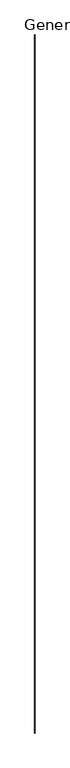
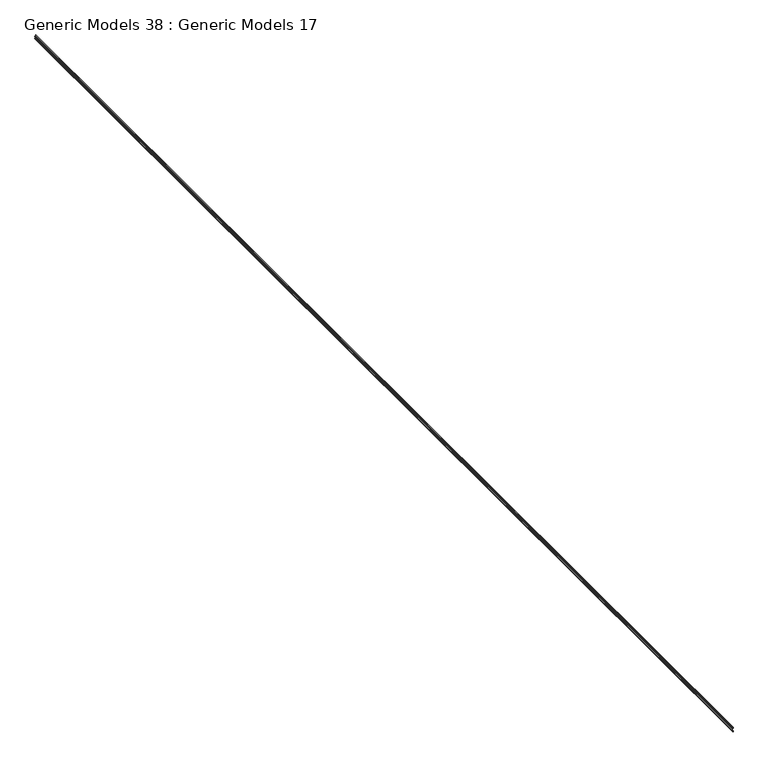
"""IFC4 building model written with IfcOpenShell, lengths in millimetres: proxy geometry, Generic Models 38 : Generic Models 17."""

from ifc_helpers import new_model, si_unit, point, frame, frame_2d, origin, place, context, project, spatial, polyline, circle_curve, trimmed, segment, composite_curve, outline, extrude, source, transform, mapped, element, save


def generic_models_38_generic_models_17_848bf92b(model_context):
    return source(origin(), model_context, "Body", "SweptSolid", [
        extrude(outline(composite_curve([segment(polyline([(266426.3089188, 23402.9215778), (266412.7835878, 23402.9215778), (266412.7835878, 23404.5090778), (266427.5844331, 23404.5090778), (266429.8980563, 23394.0193664)]), True, "CONTINUOUS"), segment(trimmed(circle_curve(frame_2d((266430.6731764, 23394.1903278)), 0.79375), [point((266429.8980563, 23394.0193664))], [point((266431.2648028, 23393.6611611))], True, "CARTESIAN"), True, "CONTINUOUS"), segment(trimmed(circle_curve(frame_2d((266434.2229343, 23391.0153278)), 3.96875), [point((266431.2648028, 23393.6611611))], [point((266434.2229343, 23394.9840778))], False, "CARTESIAN"), True, "CONTINUOUS"), segment(polyline([(266434.2229343, 23394.9840778), (266454.8442413, 23394.9840778)]), True, "CONTINUOUS"), segment(trimmed(circle_curve(frame_2d((266454.8442413, 23391.0153278)), 3.96875), [point((266454.8442413, 23394.9840778))], [point((266457.8023729, 23393.6611611))], False, "CARTESIAN"), True, "CONTINUOUS"), segment(trimmed(circle_curve(frame_2d((266458.3939992, 23394.1903278)), 0.79375), [point((266457.8023729, 23393.6611611))], [point((266459.1691194, 23394.0193664))], True, "CARTESIAN"), True, "CONTINUOUS"), segment(polyline([(266459.1691194, 23394.0193664), (266461.4827425, 23404.5090778), (266476.2835878, 23404.5090778), (266476.2835878, 23402.9215778), (266462.7582569, 23402.9215778), (266460.7193597, 23393.6774436)]), True, "CONTINUOUS"), segment(trimmed(circle_curve(frame_2d((266458.3939992, 23394.1903278)), 2.38125), [point((266460.7193597, 23393.6774436))], [point((266456.6191202, 23392.6028278))], False, "CARTESIAN"), True, "CONTINUOUS"), segment(trimmed(circle_curve(frame_2d((266454.8442413, 23391.0153278)), 2.38125), [point((266456.6191202, 23392.6028278))], [point((266454.8442413, 23393.3965778))], True, "CARTESIAN"), True, "CONTINUOUS"), segment(polyline([(266454.8442413, 23393.3965778), (266434.2229343, 23393.3965778)]), True, "CONTINUOUS"), segment(trimmed(circle_curve(frame_2d((266434.2229343, 23391.0153278)), 2.38125), [point((266434.2229343, 23393.3965778))], [point((266432.4480554, 23392.6028278))], True, "CARTESIAN"), True, "CONTINUOUS"), segment(trimmed(circle_curve(frame_2d((266430.6731764, 23394.1903278)), 2.38125), [point((266432.4480554, 23392.6028278))], [point((266428.347816, 23393.6774436))], False, "CARTESIAN"), True, "CONTINUOUS"), segment(polyline([(266428.347816, 23393.6774436), (266426.3089188, 23402.9215778)]), True, "CONTINUOUS")], self_intersect=False)), frame((0.0, 25580.0406612, 0.0), z_axis=(0.0, 1.0, 0.0), x_axis=(0.0, 0.0, 1.0)), (0.0, 0.0, 1.0), 15400.81375),
    ])


if __name__ == "__main__":
    model = new_model("IFC4")
    model_context = context("Model", 3, world=origin())
    ifc_project = project(units=[si_unit("LENGTHUNIT", "METRE", prefix="MILLI")], contexts=[model_context])
    site = spatial("IfcSite", under=ifc_project)
    building = spatial("IfcBuilding", under=site)
    placement = place(None, origin())
    generic_models_38_generic_models_17_shape = generic_models_38_generic_models_17_848bf92b(model_context)
    element("IfcBuildingElementProxy", 1, Name="Generic Models 38 : Generic Models 17", ObjectType="Generic Models 38 : Generic Models 17", at=placement, inside=building, context=model_context, shape_type="MappedRepresentation", body=[
        mapped(generic_models_38_generic_models_17_shape, transform((0.0, 0.0, 0.0), x_axis=(1.0, 0.0, 0.0), y_axis=(0.0, 1.0, 0.0), z_axis=(0.0, 0.0, 1.0))),
    ])
    save(model, "model.ifc")

# Revit data of these elements
# Element 1 (IfcBuildingElementProxy, "Generic Models 38 : Generic Models 17")
#   Materials on its faces: "1/2\" DEEP GALV. HORTZ. HAT CHANNEL @ XX O.C."
# Materials
#   "1/2\" DEEP GALV. HORTZ. HAT CHANNEL @ XX O.C.": class "Generic", colour RGB 212 212 212, transparency 0, Cost = 0
